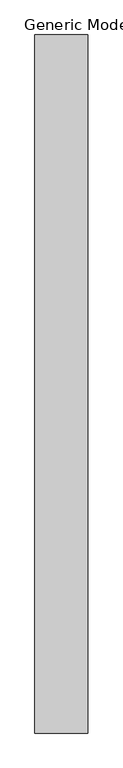
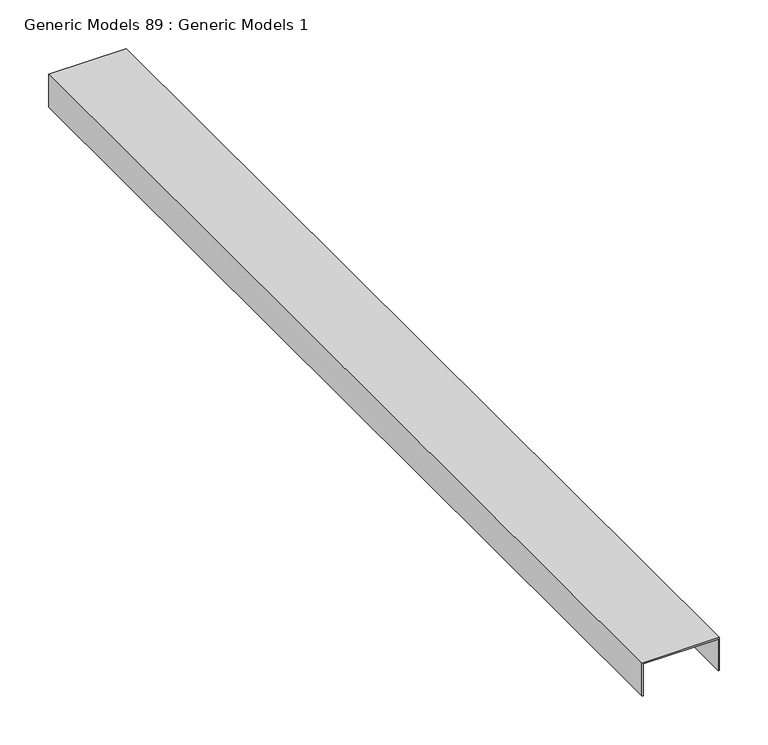
"""IFC4 building model written with IfcOpenShell, lengths in millimetres: proxy geometry, Generic Models 89 : Generic Models 1."""

from ifc_helpers import new_model, si_unit, frame, origin, place, context, project, spatial, polyline, outline, extrude, source, transform, mapped, element, save


def generic_models_89_generic_models_1_86fe7b68(model_context):
    return source(origin(), model_context, "Body", "SweptSolid", [
        extrude(outline(polyline([(2218.773933, 45716.6735531), (2218.773933, 45624.5985531), (2177.498933, 45624.5985531), (2177.498933, 45626.1860531), (2217.186433, 45626.1860531), (2217.186433, 45715.0860531), (2177.498933, 45715.0860531), (2177.498933, 45716.6735531), (2218.773933, 45716.6735531)])), frame((0.0, 0.0, 0.0), z_axis=(0.0, 1.0, 0.0), x_axis=(0.0, 0.0, 1.0)), (0.0, 0.0, 1.0), 1219.2),
    ])


if __name__ == "__main__":
    model = new_model("IFC4")
    model_context = context("Model", 3, world=origin())
    ifc_project = project(units=[si_unit("LENGTHUNIT", "METRE", prefix="MILLI")], contexts=[model_context])
    site = spatial("IfcSite", under=ifc_project)
    building = spatial("IfcBuilding", under=site)
    placement = place(None, origin())
    generic_models_89_generic_models_1_shape = generic_models_89_generic_models_1_86fe7b68(model_context)
    element("IfcBuildingElementProxy", 1, Name="Generic Models 89 : Generic Models 1", ObjectType="Generic Models 89 : Generic Models 1", at=placement, inside=building, context=model_context, shape_type="MappedRepresentation", body=[
        mapped(generic_models_89_generic_models_1_shape, transform((0.0, 0.0, 0.0), x_axis=(1.0, 0.0, 0.0), y_axis=(0.0, 1.0, 0.0), z_axis=(0.0, 0.0, 1.0))),
    ])
    save(model, "model.ifc")

# Revit data of these elements
# Element 1 (IfcBuildingElementProxy, "Generic Models 89 : Generic Models 1")
#   Materials on its faces: "METAL RUNNER CHANNEL TO RUN CONTINOUS FROM WALL TO WALL (ANCHOR AT BOTH ENDS)"
# Materials
#   "METAL RUNNER CHANNEL TO RUN CONTINOUS FROM WALL TO WALL (ANCHOR AT BOTH ENDS)": class "Unassigned", colour RGB 210 209 208, transparency 0, Keynote = "M05121300.02", Cost = 0
